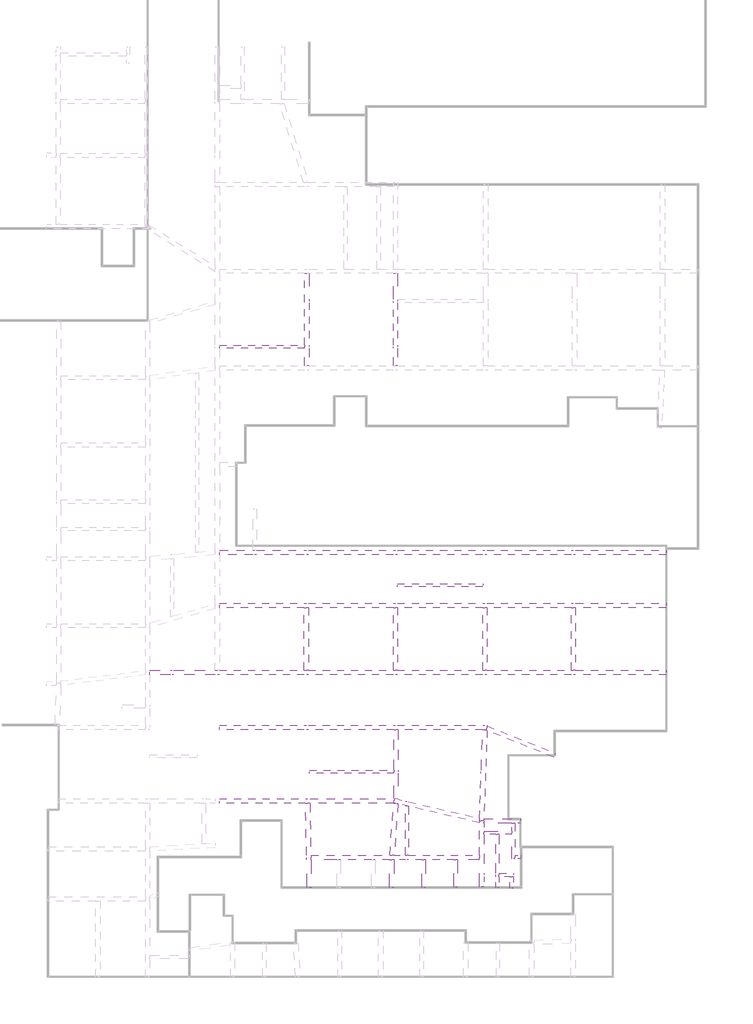
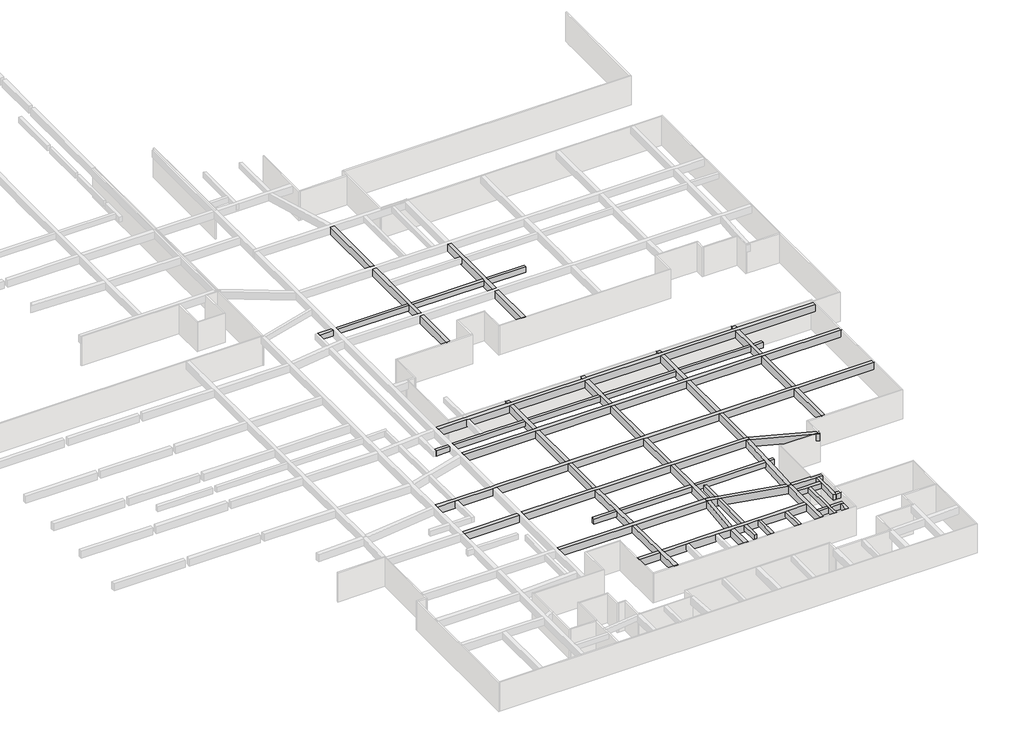
# One storey, part 10 of 16: 33 beams.
"""IFC4 building model written with IfcOpenShell, lengths in millimetres."""

from ifc_helpers import new_model, si_unit, frame, origin, place, context, project, spatial, polyline, outline, extrude, faceted_brep, element, save

model = new_model("IFC4")

# Units and contexts
model_context = context("Model", 3, world=origin())
ifc_project = project(units=[si_unit("LENGTHUNIT", "METRE", prefix="MILLI")], contexts=[model_context])

# Site, building, storey
site = spatial("IfcSite", under=ifc_project)
building = spatial("IfcBuilding", under=site)
storey = spatial("IfcBuildingStorey", under=building, Name="户型图", Elevation=0.0)

# Beams
placement = place(None, origin())
element("IfcBeam", 1, ObjectType="混凝土 - 矩形梁 : KL_beam", at=placement, inside=storey, context=model_context, shape_type="Brep", body=[
    faceted_brep([(196655.472134, 110111.2603451, 3300.0), (196255.472134, 110111.2603451, 3300.0), (196255.472134, 110111.2603451, 2500.0), (196655.472134, 110111.2603451, 2500.0), (196655.472134, 115130.098028, 3300.0), (196255.472134, 115130.098028, 3300.0), (196255.472134, 115130.098028, 2500.0), (196655.472134, 115130.098028, 2500.0)], [[[0, 1, 2, 3]], [[1, 0, 4, 5]], [[2, 1, 5, 6]], [[3, 2, 6, 7]], [[0, 3, 7, 4]], [[5, 4, 7, 6]]]),
    faceted_brep([(196255.472134, 123932.2101355, 3300.0), (196655.472134, 123932.2101355, 3300.0), (196655.472134, 123932.2101355, 2500.0), (196255.472134, 123932.2101355, 2500.0), (196655.472134, 115530.098028, 3300.0), (196255.472134, 115530.098028, 3300.0), (196255.472134, 115530.098028, 2500.0), (196655.472134, 115530.098028, 2500.0), (196255.472134, 117415.9096032, 3300.0), (196255.472134, 117115.9096032, 3300.0), (196655.472134, 117115.9096032, 3300.0), (196655.472134, 117415.9096032, 3300.0), (196655.472134, 121262.5884701, 3300.0), (196655.472134, 121562.5884701, 3300.0)], [[[0, 1, 2, 3]], [[4, 5, 6, 7]], [[1, 0, 8, 9, 5, 4, 10, 11, 12, 13]], [[0, 3, 6, 5, 9, 8]], [[3, 2, 7, 6]], [[2, 1, 13, 12, 11, 10, 4, 7]]]),
    faceted_brep([(196655.472134, 124332.2101355, 3300.0), (196255.472134, 124332.2101355, 3300.0), (196255.472134, 124332.2101355, 2500.0), (196655.472134, 124332.2101355, 2500.0), (196655.472134, 131811.3072201, 3300.0), (196255.472134, 131811.3072201, 3300.0), (196255.472134, 131811.3072201, 2500.0), (196655.472134, 131811.3072201, 2500.0)], [[[0, 1, 2, 3]], [[1, 0, 4, 5]], [[2, 1, 5, 6]], [[3, 2, 6, 7]], [[0, 3, 7, 4]], [[5, 4, 7, 6]]]),
])
element("IfcBeam", 2, ObjectType="混凝土 - 矩形梁 : KL_beam", at=placement, inside=storey, context=model_context, shape_type="Brep", body=[
    faceted_brep([(204716.2109037, 110061.7113145, 3300.0), (204316.2109037, 110061.7113145, 3300.0), (204316.2109037, 110061.7113145, 2500.0), (204716.2109037, 110061.7113145, 2500.0), (204716.2109037, 115130.098028, 3300.0), (204316.2109037, 115130.098028, 3300.0), (204316.2109037, 115130.098028, 2500.0), (204716.2109037, 115130.098028, 2500.0)], [[[0, 1, 2, 3]], [[1, 0, 4, 5]], [[2, 1, 5, 6]], [[3, 2, 6, 7]], [[0, 3, 7, 4]], [[5, 4, 7, 6]]]),
    faceted_brep([(204316.2109037, 123932.2101355, 3300.0), (204716.2109037, 123932.2101355, 3300.0), (204716.2109037, 123932.2101355, 2500.0), (204316.2109037, 123932.2101355, 2500.0), (204716.2109037, 115530.098028, 3300.0), (204316.2109037, 115530.098028, 3300.0), (204316.2109037, 115530.098028, 2500.0), (204716.2109037, 115530.098028, 2500.0), (204316.2109037, 121562.5884701, 3300.0), (204316.2109037, 121262.5884701, 3300.0), (204316.2109037, 117415.9096032, 3300.0), (204316.2109037, 117115.9096032, 3300.0), (204716.2109037, 117115.9096032, 3300.0), (204716.2109037, 117415.9096032, 3300.0), (204716.2109037, 121262.5884701, 3300.0), (204716.2109037, 121562.5884701, 3300.0)], [[[0, 1, 2, 3]], [[4, 5, 6, 7]], [[1, 0, 8, 9, 10, 11, 5, 4, 12, 13, 14, 15]], [[0, 3, 6, 5, 11, 10, 9, 8]], [[3, 2, 7, 6]], [[2, 1, 15, 14, 13, 12, 4, 7]]]),
])
element("IfcBeam", 3, ObjectType="混凝土 - 矩形梁 : KL_beam", at=placement, inside=storey, context=model_context, shape_type="Brep", body=[
    faceted_brep([(229165.989453, 87831.9011327, 3300.0), (229165.989453, 87431.9011327, 3300.0), (229165.989453, 87431.9011327, 2500.0), (229165.989453, 87831.9011327, 2500.0), (220916.2109037, 87831.9011327, 3300.0), (220516.2109037, 87831.9011327, 3300.0), (212857.7367524, 87831.9011327, 3300.0), (212457.7367524, 87831.9011327, 3300.0), (204716.2109037, 87831.9011327, 3300.0), (204316.2109037, 87831.9011327, 3300.0), (196616.2109037, 87831.9011327, 3300.0), (196216.2109037, 87831.9011327, 3300.0), (188516.2109037, 87831.9011327, 3300.0), (188116.2109037, 87831.9011327, 3300.0), (184337.9237533, 87831.9011327, 3300.0), (184037.9237533, 87831.9011327, 3300.0), (182157.7367524, 87831.9011327, 3300.0), (182157.7367524, 87431.9011327, 3300.0), (184037.9237533, 87431.9011327, 3300.0), (184337.9237533, 87431.9011327, 3300.0), (188116.2109037, 87431.9011327, 3300.0), (188516.2109037, 87431.9011327, 3300.0), (196216.2109037, 87431.9011327, 3300.0), (196616.2109037, 87431.9011327, 3300.0), (204316.2109037, 87431.9011327, 3300.0), (204716.2109037, 87431.9011327, 3300.0), (212457.7367524, 87431.9011327, 3300.0), (212857.7367524, 87431.9011327, 3300.0), (220516.2109037, 87431.9011327, 3300.0), (220916.2109037, 87431.9011327, 3300.0), (182157.7367524, 87431.9011327, 2500.0), (188116.2109037, 87431.9011327, 2500.0), (188516.2109037, 87431.9011327, 2500.0), (196216.2109037, 87431.9011327, 2500.0), (196616.2109037, 87431.9011327, 2500.0), (204316.2109037, 87431.9011327, 2500.0), (204716.2109037, 87431.9011327, 2500.0), (212457.7367524, 87431.9011327, 2500.0), (212857.7367524, 87431.9011327, 2500.0), (220516.2109037, 87431.9011327, 2500.0), (220916.2109037, 87431.9011327, 2500.0), (182157.7367524, 87831.9011327, 2500.0), (188116.2109037, 87831.9011327, 2500.0), (188516.2109037, 87831.9011327, 2500.0), (196216.2109037, 87831.9011327, 2500.0), (196616.2109037, 87831.9011327, 2500.0), (204316.2109037, 87831.9011327, 2500.0), (204716.2109037, 87831.9011327, 2500.0), (212457.7367524, 87831.9011327, 2500.0), (212857.7367524, 87831.9011327, 2500.0), (220516.2109037, 87831.9011327, 2500.0), (220916.2109037, 87831.9011327, 2500.0)], [[[0, 1, 2, 3]], [[1, 0, 4, 5, 6, 7, 8, 9, 10, 11, 12, 13, 14, 15, 16, 17, 18, 19, 20, 21, 22, 23, 24, 25, 26, 27, 28, 29]], [[2, 1, 29, 28, 27, 26, 25, 24, 23, 22, 21, 20, 19, 18, 17, 30, 31, 32, 33, 34, 35, 36, 37, 38, 39, 40]], [[3, 2, 40, 39, 38, 37, 36, 35, 34, 33, 32, 31, 30, 41, 42, 43, 44, 45, 46, 47, 48, 49, 50, 51]], [[0, 3, 51, 50, 49, 48, 47, 46, 45, 44, 43, 42, 41, 16, 15, 14, 13, 12, 11, 10, 9, 8, 7, 6, 5, 4]], [[17, 16, 41, 30]]]),
])
element("IfcBeam", 4, ObjectType="混凝土 - 矩形梁 : KL_beam", at=placement, inside=storey, context=model_context, shape_type="Brep", body=[
    faceted_brep([(229166.3202787, 93928.4104182, 3300.0), (229166.3202787, 93528.4104182, 3300.0), (229166.3202787, 93528.4104182, 2500.0), (229166.3202787, 93928.4104182, 2500.0), (220916.2109037, 93928.4104182, 3300.0), (220516.2109037, 93928.4104182, 3300.0), (212857.7367524, 93928.4104182, 3300.0), (212457.7367524, 93928.4104182, 3300.0), (204716.2109037, 93928.4104182, 3300.0), (204316.2109037, 93928.4104182, 3300.0), (196616.2109037, 93928.4104182, 3300.0), (196216.2109037, 93928.4104182, 3300.0), (188516.2109037, 93928.4104182, 3300.0), (188516.2109037, 93528.4104182, 3300.0), (196216.2109037, 93528.4104182, 3300.0), (196616.2109037, 93528.4104182, 3300.0), (204316.2109037, 93528.4104182, 3300.0), (204716.2109037, 93528.4104182, 3300.0), (212457.7367524, 93528.4104182, 3300.0), (212857.7367524, 93528.4104182, 3300.0), (220516.2109037, 93528.4104182, 3300.0), (220916.2109037, 93528.4104182, 3300.0), (188516.2109037, 93528.4104182, 2500.0), (196216.2109037, 93528.4104182, 2500.0), (196616.2109037, 93528.4104182, 2500.0), (204316.2109037, 93528.4104182, 2500.0), (204716.2109037, 93528.4104182, 2500.0), (212457.7367524, 93528.4104182, 2500.0), (212857.7367524, 93528.4104182, 2500.0), (220516.2109037, 93528.4104182, 2500.0), (220916.2109037, 93528.4104182, 2500.0), (188516.2109037, 93928.4104182, 2500.0), (196216.2109037, 93928.4104182, 2500.0), (196616.2109037, 93928.4104182, 2500.0), (204316.2109037, 93928.4104182, 2500.0), (204716.2109037, 93928.4104182, 2500.0), (212457.7367524, 93928.4104182, 2500.0), (212857.7367524, 93928.4104182, 2500.0), (220516.2109037, 93928.4104182, 2500.0), (220916.2109037, 93928.4104182, 2500.0)], [[[0, 1, 2, 3]], [[1, 0, 4, 5, 6, 7, 8, 9, 10, 11, 12, 13, 14, 15, 16, 17, 18, 19, 20, 21]], [[2, 1, 21, 20, 19, 18, 17, 16, 15, 14, 13, 22, 23, 24, 25, 26, 27, 28, 29, 30]], [[3, 2, 30, 29, 28, 27, 26, 25, 24, 23, 22, 31, 32, 33, 34, 35, 36, 37, 38, 39]], [[0, 3, 39, 38, 37, 36, 35, 34, 33, 32, 31, 12, 11, 10, 9, 8, 7, 6, 5, 4]], [[12, 31, 22, 13]]]),
])
element("IfcBeam", 5, ObjectType="混凝土 - 矩形梁 : KL_beam", at=placement, inside=storey, context=model_context, shape_type="Brep", body=[
    faceted_brep([(229166.2265287, 98740.0727237, 3300.0), (229166.2265287, 98340.0727237, 3300.0), (229166.2265287, 98340.0727237, 2500.0), (229166.2265287, 98740.0727237, 2500.0), (220916.2109037, 98740.0727237, 3300.0), (220516.2109037, 98740.0727237, 3300.0), (212857.7367524, 98740.0727237, 3300.0), (212457.7367524, 98740.0727237, 3300.0), (204716.2109037, 98740.0727237, 3300.0), (204316.2109037, 98740.0727237, 3300.0), (196616.2109037, 98740.0727237, 3300.0), (196216.2109037, 98740.0727237, 3300.0), (191866.2868684, 98740.0727237, 3300.0), (191566.2868684, 98740.0727237, 3300.0), (188516.2109037, 98740.0727237, 3300.0), (188516.2109037, 98340.0727237, 3300.0), (191566.2868684, 98340.0727237, 3300.0), (191866.2868684, 98340.0727237, 3300.0), (196216.2109037, 98340.0727237, 3300.0), (196616.2109037, 98340.0727237, 3300.0), (204316.2109037, 98340.0727237, 3300.0), (204716.2109037, 98340.0727237, 3300.0), (212457.7367524, 98340.0727237, 3300.0), (212857.7367524, 98340.0727237, 3300.0), (220516.2109037, 98340.0727237, 3300.0), (220916.2109037, 98340.0727237, 3300.0), (188516.2109037, 98340.0727237, 2500.0), (196216.2109037, 98340.0727237, 2500.0), (196616.2109037, 98340.0727237, 2500.0), (204316.2109037, 98340.0727237, 2500.0), (204716.2109037, 98340.0727237, 2500.0), (212457.7367524, 98340.0727237, 2500.0), (212857.7367524, 98340.0727237, 2500.0), (220516.2109037, 98340.0727237, 2500.0), (220916.2109037, 98340.0727237, 2500.0), (188516.2109037, 98740.0727237, 2500.0), (196216.2109037, 98740.0727237, 2500.0), (196616.2109037, 98740.0727237, 2500.0), (204316.2109037, 98740.0727237, 2500.0), (204716.2109037, 98740.0727237, 2500.0), (212457.7367524, 98740.0727237, 2500.0), (212857.7367524, 98740.0727237, 2500.0), (220516.2109037, 98740.0727237, 2500.0), (220916.2109037, 98740.0727237, 2500.0)], [[[0, 1, 2, 3]], [[1, 0, 4, 5, 6, 7, 8, 9, 10, 11, 12, 13, 14, 15, 16, 17, 18, 19, 20, 21, 22, 23, 24, 25]], [[2, 1, 25, 24, 23, 22, 21, 20, 19, 18, 17, 16, 15, 26, 27, 28, 29, 30, 31, 32, 33, 34]], [[3, 2, 34, 33, 32, 31, 30, 29, 28, 27, 26, 35, 36, 37, 38, 39, 40, 41, 42, 43]], [[0, 3, 43, 42, 41, 40, 39, 38, 37, 36, 35, 14, 13, 12, 11, 10, 9, 8, 7, 6, 5, 4]], [[14, 35, 26, 15]]]),
])
element("IfcBeam", 6, ObjectType="混凝土 - 矩形梁 : KL_beam", at=placement, inside=storey, context=model_context, shape_type="Brep", body=[
    faceted_brep([(212857.7367524, 82438.0259701, 3300.0), (212857.7367524, 82773.7000033, 3300.0), (212857.7367524, 82838.0259701, 3300.0), (212457.7367524, 82838.0259701, 3300.0), (204716.2109037, 82838.0259701, 3300.0), (204316.2109037, 82838.0259701, 3300.0), (196616.2109037, 82838.0259701, 3300.0), (196216.2109037, 82838.0259701, 3300.0), (188516.2109037, 82838.0259701, 3300.0), (188516.2109037, 82438.0259701, 3300.0), (196219.671451, 82438.0259701, 3300.0), (196619.7323823, 82438.0259701, 3300.0), (204365.5652507, 82438.0259701, 3300.0), (204765.5652507, 82438.0259701, 3300.0), (212450.6306897, 82438.0259701, 3300.0), (212619.4103045, 82438.0259701, 3300.0), (212857.7367524, 82438.0259701, 2500.0), (188516.2109037, 82438.0259701, 2500.0), (196219.671451, 82438.0259701, 2500.0), (196619.7323823, 82438.0259701, 2500.0), (204365.5652507, 82438.0259701, 2500.0), (204765.5652507, 82438.0259701, 2500.0), (212450.6306897, 82438.0259701, 2500.0), (212619.4103045, 82438.0259701, 2500.0), (212857.7367524, 82838.0259701, 2500.0), (212857.7367524, 82773.7000033, 2500.0), (188516.2109037, 82838.0259701, 2500.0), (196216.2109037, 82838.0259701, 2500.0), (196616.2109037, 82838.0259701, 2500.0), (204316.2109037, 82838.0259701, 2500.0), (204716.2109037, 82838.0259701, 2500.0), (212457.7367524, 82838.0259701, 2500.0)], [[[0, 1, 2, 3, 4, 5, 6, 7, 8, 9, 10, 11, 12, 13, 14, 15]], [[16, 0, 15, 14, 13, 12, 11, 10, 9, 17, 18, 19, 20, 21, 22, 23]], [[24, 25, 16, 23, 22, 21, 20, 19, 18, 17, 26, 27, 28, 29, 30, 31]], [[2, 24, 31, 30, 29, 28, 27, 26, 8, 7, 6, 5, 4, 3]], [[9, 8, 26, 17]], [[2, 1, 0, 16, 25, 24]]]),
    faceted_brep([(182157.7367524, 82438.0259701, 3300.0), (182157.7367524, 82838.0259701, 3300.0), (182157.7367524, 82838.0259701, 2500.0), (182157.7367524, 82438.0259701, 2500.0), (188116.2109037, 82838.0259701, 3300.0), (188116.2109037, 82438.0259701, 3300.0), (188116.2109037, 82438.0259701, 2500.0), (188116.2109037, 82838.0259701, 2500.0)], [[[0, 1, 2, 3]], [[4, 5, 6, 7]], [[1, 0, 5, 4]], [[0, 3, 6, 5]], [[3, 2, 7, 6]], [[2, 1, 4, 7]]]),
])
element("IfcBeam", 7, ObjectType="混凝土 - 矩形梁 : KL_beam", at=placement, inside=storey, context=model_context, shape_type="Brep", body=[
    faceted_brep([(196216.2109037, 99161.1613461, 3300.0), (196616.2109037, 99161.1613461, 3300.0), (196616.2109037, 99161.1613461, 2500.0), (196216.2109037, 99161.1613461, 2500.0), (196216.2109037, 98740.0727237, 3300.0), (196616.2109037, 98740.0727237, 3300.0), (196616.2109037, 98740.0727237, 2500.0), (196216.2109037, 98740.0727237, 2500.0)], [[[0, 1, 2, 3]], [[1, 0, 4, 5]], [[2, 1, 5, 6]], [[3, 2, 6, 7]], [[0, 3, 7, 4]], [[5, 4, 7, 6]]]),
    faceted_brep([(196616.2109037, 82838.0259701, 3300.0), (196216.2109037, 82838.0259701, 3300.0), (196216.2109037, 82838.0259701, 2500.0), (196616.2109037, 82838.0259701, 2500.0), (196216.2109037, 87431.9011327, 3300.0), (196616.2109037, 87431.9011327, 3300.0), (196616.2109037, 87431.9011327, 2500.0), (196216.2109037, 87431.9011327, 2500.0)], [[[0, 1, 2, 3]], [[4, 5, 6, 7]], [[1, 0, 5, 4]], [[0, 3, 6, 5]], [[3, 2, 7, 6]], [[2, 1, 4, 7]]]),
    faceted_brep([(196616.2109037, 87831.9011327, 3300.0), (196216.2109037, 87831.9011327, 3300.0), (196216.2109037, 87831.9011327, 2500.0), (196616.2109037, 87831.9011327, 2500.0), (196216.2109037, 93528.4104182, 3300.0), (196616.2109037, 93528.4104182, 3300.0), (196616.2109037, 93528.4104182, 2500.0), (196216.2109037, 93528.4104182, 2500.0)], [[[0, 1, 2, 3]], [[4, 5, 6, 7]], [[1, 0, 5, 4]], [[0, 3, 6, 5]], [[3, 2, 7, 6]], [[2, 1, 4, 7]]]),
    faceted_brep([(196616.2109037, 93928.4104182, 3300.0), (196216.2109037, 93928.4104182, 3300.0), (196216.2109037, 93928.4104182, 2500.0), (196616.2109037, 93928.4104182, 2500.0), (196216.2109037, 98340.0727237, 3300.0), (196616.2109037, 98340.0727237, 3300.0), (196616.2109037, 98340.0727237, 2500.0), (196216.2109037, 98340.0727237, 2500.0), (196616.2109037, 95415.9096032, 3300.0), (196616.2109037, 95715.9096032, 3300.0), (196216.2109037, 95715.9096032, 3300.0), (196216.2109037, 95415.9096032, 3300.0)], [[[0, 1, 2, 3]], [[4, 5, 6, 7]], [[1, 0, 8, 9, 5, 4, 10, 11]], [[0, 3, 6, 5, 9, 8]], [[3, 2, 7, 6]], [[2, 1, 11, 10, 4, 7]]]),
])
element("IfcBeam", 8, ObjectType="混凝土 - 矩形梁 : KL_beam", at=placement, inside=storey, context=model_context, shape_type="Brep", body=[
    faceted_brep([(204316.2109037, 99161.1613461, 3300.0), (204716.2109037, 99161.1613461, 3300.0), (204716.2109037, 99161.1613461, 2500.0), (204316.2109037, 99161.1613461, 2500.0), (204316.2109037, 98740.0727237, 3300.0), (204716.2109037, 98740.0727237, 3300.0), (204716.2109037, 98740.0727237, 2500.0), (204316.2109037, 98740.0727237, 2500.0)], [[[0, 1, 2, 3]], [[1, 0, 4, 5]], [[2, 1, 5, 6]], [[3, 2, 6, 7]], [[0, 3, 7, 4]], [[5, 4, 7, 6]]]),
    faceted_brep([(204716.2109037, 82838.0259701, 3300.0), (204316.2109037, 82838.0259701, 3300.0), (204316.2109037, 82838.0259701, 2500.0), (204716.2109037, 82838.0259701, 2500.0), (204316.2109037, 87431.9011327, 3300.0), (204716.2109037, 87431.9011327, 3300.0), (204716.2109037, 87431.9011327, 2500.0), (204316.2109037, 87431.9011327, 2500.0)], [[[0, 1, 2, 3]], [[4, 5, 6, 7]], [[1, 0, 5, 4]], [[0, 3, 6, 5]], [[3, 2, 7, 6]], [[2, 1, 4, 7]]]),
    faceted_brep([(204716.2109037, 87831.9011327, 3300.0), (204316.2109037, 87831.9011327, 3300.0), (204316.2109037, 87831.9011327, 2500.0), (204716.2109037, 87831.9011327, 2500.0), (204316.2109037, 93528.4104182, 3300.0), (204716.2109037, 93528.4104182, 3300.0), (204716.2109037, 93528.4104182, 2500.0), (204316.2109037, 93528.4104182, 2500.0)], [[[0, 1, 2, 3]], [[4, 5, 6, 7]], [[1, 0, 5, 4]], [[0, 3, 6, 5]], [[3, 2, 7, 6]], [[2, 1, 4, 7]]]),
    faceted_brep([(204716.2109037, 93928.4104182, 3300.0), (204316.2109037, 93928.4104182, 3300.0), (204316.2109037, 93928.4104182, 2500.0), (204716.2109037, 93928.4104182, 2500.0), (204316.2109037, 98340.0727237, 3300.0), (204716.2109037, 98340.0727237, 3300.0), (204716.2109037, 98340.0727237, 2500.0), (204316.2109037, 98340.0727237, 2500.0), (204716.2109037, 95415.9096032, 3300.0), (204716.2109037, 95715.9096032, 3300.0), (204316.2109037, 95715.9096032, 3300.0), (204316.2109037, 95415.9096032, 3300.0)], [[[0, 1, 2, 3]], [[4, 5, 6, 7]], [[1, 0, 8, 9, 5, 4, 10, 11]], [[0, 3, 6, 5, 9, 8]], [[3, 2, 7, 6]], [[2, 1, 11, 10, 4, 7]]]),
])
element("IfcBeam", 9, ObjectType="混凝土 - 矩形梁 : KL_beam", at=placement, inside=storey, context=model_context, shape_type="Brep", body=[
    faceted_brep([(212457.7367524, 99161.1665951, 3300.0), (212857.7367524, 99161.1665951, 3300.0), (212857.7367524, 99161.1665951, 2500.0), (212457.7367524, 99161.1665951, 2500.0), (212457.7367524, 98740.0727237, 3300.0), (212857.7367524, 98740.0727237, 3300.0), (212857.7367524, 98740.0727237, 2500.0), (212457.7367524, 98740.0727237, 2500.0)], [[[0, 1, 2, 3]], [[1, 0, 4, 5]], [[2, 1, 5, 6]], [[3, 2, 6, 7]], [[0, 3, 7, 4]], [[5, 4, 7, 6]]]),
    faceted_brep([(212857.7367524, 82838.0259701, 3300.0), (212457.7367524, 82838.0259701, 3300.0), (212457.7367524, 82838.0259701, 2500.0), (212857.7367524, 82838.0259701, 2500.0), (212457.7367524, 87431.9011327, 3300.0), (212857.7367524, 87431.9011327, 3300.0), (212857.7367524, 87431.9011327, 2500.0), (212457.7367524, 87431.9011327, 2500.0)], [[[0, 1, 2, 3]], [[4, 5, 6, 7]], [[1, 0, 5, 4]], [[0, 3, 6, 5]], [[3, 2, 7, 6]], [[2, 1, 4, 7]]]),
    faceted_brep([(212857.7367524, 87831.9011327, 3300.0), (212457.7367524, 87831.9011327, 3300.0), (212457.7367524, 87831.9011327, 2500.0), (212857.7367524, 87831.9011327, 2500.0), (212457.7367524, 93528.4104182, 3300.0), (212857.7367524, 93528.4104182, 3300.0), (212857.7367524, 93528.4104182, 2500.0), (212457.7367524, 93528.4104182, 2500.0)], [[[0, 1, 2, 3]], [[4, 5, 6, 7]], [[1, 0, 5, 4]], [[0, 3, 6, 5]], [[3, 2, 7, 6]], [[2, 1, 4, 7]]]),
    faceted_brep([(212857.7367524, 93928.4104182, 3300.0), (212457.7367524, 93928.4104182, 3300.0), (212457.7367524, 93928.4104182, 2500.0), (212857.7367524, 93928.4104182, 2500.0), (212457.7367524, 98340.0727237, 3300.0), (212857.7367524, 98340.0727237, 3300.0), (212857.7367524, 98340.0727237, 2500.0), (212457.7367524, 98340.0727237, 2500.0), (212857.7367524, 95415.9096032, 3300.0), (212857.7367524, 95715.9096032, 3300.0), (212457.7367524, 95715.9096032, 3300.0), (212457.7367524, 95415.9096032, 3300.0)], [[[0, 1, 2, 3]], [[4, 5, 6, 7]], [[1, 0, 8, 9, 5, 4, 10, 11]], [[0, 3, 6, 5, 9, 8]], [[3, 2, 7, 6]], [[2, 1, 11, 10, 4, 7]]]),
])
element("IfcBeam", 10, ObjectType="混凝土 - 矩形梁 : KL_beam", at=placement, inside=storey, context=model_context, shape_type="Brep", body=[
    faceted_brep([(220516.2109037, 99161.2550961, 3300.0), (220916.2109037, 99161.2550961, 3300.0), (220916.2109037, 99161.2550961, 2500.0), (220516.2109037, 99161.2550961, 2500.0), (220516.2109037, 98740.0727237, 3300.0), (220916.2109037, 98740.0727237, 3300.0), (220916.2109037, 98740.0727237, 2500.0), (220516.2109037, 98740.0727237, 2500.0)], [[[0, 1, 2, 3]], [[1, 0, 4, 5]], [[2, 1, 5, 6]], [[3, 2, 6, 7]], [[0, 3, 7, 4]], [[5, 4, 7, 6]]]),
    faceted_brep([(220516.2109037, 82302.2550961, 3300.0), (220516.2109037, 82302.2550961, 2500.0), (220916.2109037, 82302.2550961, 2500.0), (220916.2109037, 82302.2550961, 3300.0), (220516.2109037, 87431.9011327, 3300.0), (220916.2109037, 87431.9011327, 3300.0), (220916.2109037, 87431.9011327, 2500.0), (220516.2109037, 87431.9011327, 2500.0)], [[[0, 1, 2, 3]], [[4, 5, 6, 7]], [[0, 3, 5, 4]], [[3, 2, 6, 5]], [[2, 1, 7, 6]], [[1, 0, 4, 7]]]),
    faceted_brep([(220916.2109037, 87831.9011327, 3300.0), (220516.2109037, 87831.9011327, 3300.0), (220516.2109037, 87831.9011327, 2500.0), (220916.2109037, 87831.9011327, 2500.0), (220516.2109037, 93528.4104182, 3300.0), (220916.2109037, 93528.4104182, 3300.0), (220916.2109037, 93528.4104182, 2500.0), (220516.2109037, 93528.4104182, 2500.0)], [[[0, 1, 2, 3]], [[4, 5, 6, 7]], [[1, 0, 5, 4]], [[0, 3, 6, 5]], [[3, 2, 7, 6]], [[2, 1, 4, 7]]]),
    faceted_brep([(220916.2109037, 93928.4104182, 3300.0), (220516.2109037, 93928.4104182, 3300.0), (220516.2109037, 93928.4104182, 2500.0), (220916.2109037, 93928.4104182, 2500.0), (220516.2109037, 98340.0727237, 3300.0), (220916.2109037, 98340.0727237, 3300.0), (220916.2109037, 98340.0727237, 2500.0), (220516.2109037, 98340.0727237, 2500.0), (220916.2109037, 95415.9096032, 3300.0), (220916.2109037, 95715.9096032, 3300.0), (220516.2109037, 95715.9096032, 3300.0), (220516.2109037, 95415.9096032, 3300.0)], [[[0, 1, 2, 3]], [[4, 5, 6, 7]], [[1, 0, 8, 9, 5, 4, 10, 11]], [[0, 3, 6, 5, 9, 8]], [[3, 2, 7, 6]], [[2, 1, 11, 10, 4, 7]]]),
])
element("IfcBeam", 11, ObjectType="混凝土 - 矩形梁 : KL_beam", at=placement, inside=storey, context=model_context, shape_type="Brep", body=[
    faceted_brep([(219079.6758919, 80298.142032, 3300.0), (218931.8005151, 79926.4797217, 3300.0), (218931.8005151, 79926.4797217, 2500.0), (219079.6758919, 80298.142032, 2500.0), (212857.7367524, 82773.7000033, 3300.0), (212857.7367524, 82438.0259701, 3300.0), (212619.4103045, 82438.0259701, 3300.0), (212847.7025863, 82347.1940341, 3300.0), (212619.4103045, 82438.0259701, 2500.0), (212847.7025863, 82347.1940341, 2500.0), (212857.7367524, 82438.0259701, 2500.0), (212857.7367524, 82773.7000033, 2500.0)], [[[0, 1, 2, 3]], [[1, 0, 4, 5, 6, 7]], [[2, 1, 7, 6, 8, 9]], [[3, 2, 9, 8, 10, 11]], [[0, 3, 11, 4]], [[5, 10, 8, 6]], [[10, 5, 4, 11]]]),
])
element("IfcBeam", 12, ObjectType="混凝土 - 矩形梁 : KL_beam", at=placement, inside=storey, context=model_context, shape_type="Brep", body=[
    faceted_brep([(212450.6306897, 82438.0259701, 3300.0), (212321.9177065, 78752.1683832, 3300.0), (212311.4414756, 78452.1683832, 3300.0), (212169.1148986, 74376.4684731, 3300.0), (212160.525769, 74130.5079832, 3300.0), (212560.525769, 74123.5259572, 3300.0), (212567.6318318, 74327.0169702, 3300.0), (212711.6852934, 78452.1683832, 3300.0), (212722.1615242, 78752.1683832, 3300.0), (212847.7025863, 82347.1940341, 3300.0), (212619.4103045, 82438.0259701, 3300.0), (212457.7367524, 82438.0259701, 3300.0), (212450.6306897, 82438.0259701, 2500.0), (212169.1148986, 74376.4684731, 2500.0), (212160.525769, 74130.5079832, 2500.0), (212457.7367524, 82438.0259701, 2500.0), (212619.4103045, 82438.0259701, 2500.0), (212847.7025863, 82347.1940341, 2500.0), (212567.6318318, 74327.0169702, 2500.0), (212560.525769, 74123.5259572, 2500.0)], [[[0, 1, 2, 3, 4, 5, 6, 7, 8, 9, 10, 11]], [[4, 3, 2, 1, 0, 12, 13, 14]], [[14, 13, 12, 15, 16, 17, 18, 19]], [[5, 19, 18, 17, 9, 8, 7, 6]], [[12, 0, 11, 10, 16, 15]], [[10, 9, 17, 16]], [[5, 4, 14, 19]]]),
])
element("IfcBeam", 13, ObjectType="混凝土 - 矩形梁 : KL_beam", at=placement, inside=storey, context=model_context, shape_type="Brep", body=[
    faceted_brep([(212560.525769, 68162.6620951, 3300.0), (212160.525769, 68162.6620951, 3300.0), (212160.525769, 68162.6620951, 2500.0), (212560.525769, 68162.6620951, 2500.0), (212560.525769, 69072.3236201, 3300.0), (212560.525769, 69372.3236201, 3300.0), (212560.525769, 72912.3072201, 3300.0), (212560.525769, 73212.3072201, 3300.0), (212560.525769, 73927.0169702, 3300.0), (212560.525769, 74123.5259572, 3300.0), (212160.525769, 74130.5079832, 3300.0), (212160.525769, 73967.9297868, 3300.0), (212160.525769, 71002.3072201, 3300.0), (212160.525769, 70602.3072201, 3300.0), (212160.525769, 74130.5079832, 2500.0), (212160.525769, 73967.9297868, 2500.0), (212160.525769, 71002.3072201, 2500.0), (212160.525769, 70602.3072201, 2500.0), (212560.525769, 74123.5259572, 2500.0), (212560.525769, 73927.0169702, 2500.0)], [[[0, 1, 2, 3]], [[1, 0, 4, 5, 6, 7, 8, 9, 10, 11, 12, 13]], [[2, 1, 13, 12, 11, 10, 14, 15, 16, 17]], [[3, 2, 17, 16, 15, 14, 18, 19]], [[0, 3, 19, 18, 9, 8, 7, 6, 5, 4]], [[9, 18, 14, 10]]]),
])
element("IfcBeam", 14, ObjectType="混凝土 - 矩形梁 : KL_beam", at=placement, inside=storey, context=model_context, shape_type="Brep", body=[
    faceted_brep([(212160.525769, 74130.5079832, 3300.0), (212169.1148986, 74376.4684731, 3300.0), (205715.469601, 75866.4098892, 3300.0), (205415.469601, 75935.6703465, 3300.0), (204765.5652507, 76085.7125882, 3300.0), (204365.5652507, 76178.0598647, 3300.0), (204365.5652507, 76126.6254049, 3300.0), (204365.5652507, 75767.5382216, 3300.0), (204542.7781291, 75726.6254049, 3300.0), (204747.7405268, 75679.3061069, 3300.0), (205415.469601, 75525.1487034, 3300.0), (205715.469601, 75455.888246, 3300.0), (212160.525769, 73967.9297868, 3300.0), (212169.1148986, 74376.4684731, 2500.0), (204765.5652507, 76085.7125882, 2500.0), (204365.5652507, 76178.0598647, 2500.0), (212160.525769, 74130.5079832, 2500.0), (212160.525769, 73967.9297868, 2500.0), (204747.7405268, 75679.3061069, 2500.0), (204542.7781291, 75726.6254049, 2500.0), (204365.5652507, 75767.5382216, 2500.0), (204365.5652507, 76126.6254049, 2500.0)], [[[0, 1, 2, 3, 4, 5, 6, 7, 8, 9, 10, 11, 12]], [[1, 13, 14, 15, 5, 4, 3, 2]], [[13, 16, 17, 18, 19, 20, 21, 15, 14]], [[7, 20, 19, 18, 17, 12, 11, 10, 9, 8]], [[1, 0, 16, 13]], [[0, 12, 17, 16]], [[7, 6, 5, 15, 21, 20]]]),
])
element("IfcBeam", 15, ObjectType="混凝土 - 矩形梁 : KL_beam", at=placement, inside=storey, context=model_context, shape_type="Brep", body=[
    faceted_brep([(204365.5652507, 76178.0598647, 3300.0), (204765.5652507, 76085.7125882, 3300.0), (204765.5652507, 78452.1683832, 3300.0), (204765.5652507, 78752.1683832, 3300.0), (204765.5652507, 82438.0259701, 3300.0), (204365.5652507, 82438.0259701, 3300.0), (204365.5652507, 78752.1683832, 3300.0), (204365.5652507, 78452.1683832, 3300.0), (204765.5652507, 76085.7125882, 2500.0), (204765.5652507, 82438.0259701, 2500.0), (204365.5652507, 76178.0598647, 2500.0), (204365.5652507, 82438.0259701, 2500.0)], [[[0, 1, 2, 3, 4, 5, 6, 7]], [[1, 8, 9, 4, 3, 2]], [[8, 10, 11, 9]], [[10, 0, 7, 6, 5, 11]], [[1, 0, 10, 8]], [[5, 4, 9, 11]]]),
])
element("IfcBeam", 16, ObjectType="混凝土 - 矩形梁 : KL_beam", at=placement, inside=storey, context=model_context, shape_type="Brep", body=[
    faceted_brep([(204542.7781291, 75726.6254049, 3300.0), (204365.5652507, 75767.5382216, 3300.0), (204365.5652507, 76126.6254049, 3300.0), (196729.8982889, 76126.6254049, 3300.0), (196329.8373577, 76126.6254049, 3300.0), (188516.2109037, 76126.6254049, 3300.0), (188516.2109037, 75726.6254049, 3300.0), (196336.8193837, 75726.6254049, 3300.0), (196736.8803149, 75726.6254049, 3300.0), (204350.1537866, 75726.6254049, 3300.0), (204365.5652507, 76126.6254049, 2500.0), (196729.8982889, 76126.6254049, 2500.0), (196329.8373577, 76126.6254049, 2500.0), (188516.2109037, 76126.6254049, 2500.0), (204365.5652507, 75767.5382216, 2500.0), (204542.7781291, 75726.6254049, 2500.0), (204350.1537866, 75726.6254049, 2500.0), (196736.8803149, 75726.6254049, 2500.0), (196336.8193837, 75726.6254049, 2500.0), (188516.2109037, 75726.6254049, 2500.0)], [[[0, 1, 2, 3, 4, 5, 6, 7, 8, 9]], [[2, 10, 11, 12, 13, 5, 4, 3]], [[14, 15, 16, 17, 18, 19, 13, 12, 11, 10]], [[15, 0, 9, 8, 7, 6, 19, 18, 17, 16]], [[14, 1, 0, 15]], [[1, 14, 10, 2]], [[6, 5, 13, 19]]]),
])
element("IfcBeam", 17, ObjectType="混凝土 - 矩形梁 : KL_beam", at=placement, inside=storey, context=model_context, shape_type="Brep", body=[
    faceted_brep([(196870.5923656, 68066.2671502, 3300.0), (196470.6532875, 68059.2861877, 3300.0), (196470.6532875, 68059.2861877, 2500.0), (196870.5923656, 68066.2671502, 2500.0), (196826.3256215, 70602.3072201, 3300.0), (196819.3435955, 71002.3072201, 3300.0), (196736.8803149, 75726.6254049, 3300.0), (196336.8193837, 75726.6254049, 3300.0), (196419.2826643, 71002.3072201, 3300.0), (196426.2646903, 70602.3072201, 3300.0), (196336.8193837, 75726.6254049, 2500.0), (196419.2826643, 71002.3072201, 2500.0), (196426.2646903, 70602.3072201, 2500.0), (196736.8803149, 75726.6254049, 2500.0), (196819.3435955, 71002.3072201, 2500.0), (196826.3256215, 70602.3072201, 2500.0)], [[[0, 1, 2, 3]], [[1, 0, 4, 5, 6, 7, 8, 9]], [[2, 1, 9, 8, 7, 10, 11, 12]], [[3, 2, 12, 11, 10, 13, 14, 15]], [[0, 3, 15, 14, 13, 6, 5, 4]], [[7, 6, 13, 10]]]),
    faceted_brep([(196219.671451, 82438.0259701, 3300.0), (196619.7323823, 82438.0259701, 3300.0), (196619.7323823, 82438.0259701, 2500.0), (196219.671451, 82438.0259701, 2500.0), (196729.8982889, 76126.6254049, 3300.0), (196329.8373577, 76126.6254049, 3300.0), (196329.8373577, 76126.6254049, 2500.0), (196729.8982889, 76126.6254049, 2500.0), (196284.0083345, 78752.1683832, 3300.0), (196289.244854, 78452.1683832, 3300.0), (196689.3057852, 78452.1683832, 3300.0), (196684.0692657, 78752.1683832, 3300.0)], [[[0, 1, 2, 3]], [[4, 5, 6, 7]], [[1, 0, 8, 9, 5, 4, 10, 11]], [[0, 3, 6, 5, 9, 8]], [[3, 2, 7, 6]], [[2, 1, 11, 10, 4, 7]]]),
])
element("IfcBeam", 18, ObjectType="混凝土 - 矩形梁 : KL_beam", at=placement, inside=storey, context=model_context, shape_type="SweptSolid", body=[
    extrude(outline(polyline([(204542.7781291, 75726.6254049), (204747.7405268, 75679.3061069), (204400.2357023, 71002.3072201), (203999.1330998, 71002.3072201), (204350.1537866, 75726.6254049), (204542.7781291, 75726.6254049)])), frame((0.0, 0.0, 2500.0), z_axis=(0.0, 0.0, 1.0), x_axis=(1.0, 0.0, 0.0)), (0.0, 0.0, 1.0), 800.0),
])
element("IfcBeam", 19, ObjectType="混凝土 - 矩形梁 : KL_beam", at=placement, inside=storey, context=model_context, shape_type="SweptSolid", body=[
    extrude(outline(polyline([(204396.7123685, 68062.3072201), (203996.7123685, 68062.3072201), (203996.7123685, 70602.3072201), (204396.7123685, 70602.3072201), (204396.7123685, 68062.3072201)])), frame((0.0, 0.0, 2500.0), z_axis=(0.0, 0.0, 1.0), x_axis=(1.0, 0.0, 0.0)), (0.0, 0.0, 1.0), 800.0),
])
element("IfcBeam", 20, ObjectType="混凝土 - 矩形梁 : KL_beam", at=placement, inside=storey, context=model_context, shape_type="Brep", body=[
    faceted_brep([(194147.1180922, 71002.3072201, 3300.0), (194147.1180922, 71002.3072201, 2500.0), (194147.1180922, 70602.3072201, 2500.0), (194147.1180922, 70602.3072201, 3300.0), (196419.2826643, 71002.3072201, 3300.0), (196426.2646903, 70602.3072201, 3300.0), (196426.2646903, 70602.3072201, 2500.0), (196419.2826643, 71002.3072201, 2500.0)], [[[0, 1, 2, 3]], [[4, 5, 6, 7]], [[0, 3, 5, 4]], [[3, 2, 6, 5]], [[2, 1, 7, 6]], [[1, 0, 4, 7]]]),
    faceted_brep([(212160.525769, 70602.3072201, 3300.0), (212160.525769, 71002.3072201, 3300.0), (205715.469601, 71002.3072201, 3300.0), (205415.469601, 71002.3072201, 3300.0), (204400.2357023, 71002.3072201, 3300.0), (203999.1330998, 71002.3072201, 3300.0), (196819.3435955, 71002.3072201, 3300.0), (196826.3256215, 70602.3072201, 3300.0), (199196.7123685, 70602.3072201, 3300.0), (199496.7123685, 70602.3072201, 3300.0), (202346.7123685, 70602.3072201, 3300.0), (202646.7123685, 70602.3072201, 3300.0), (203996.7123685, 70602.3072201, 3300.0), (204396.7123685, 70602.3072201, 3300.0), (205415.469601, 70602.3072201, 3300.0), (205715.469601, 70602.3072201, 3300.0), (206946.7123685, 70602.3072201, 3300.0), (207246.7123685, 70602.3072201, 3300.0), (209846.7143216, 70602.3072201, 3300.0), (210146.7143216, 70602.3072201, 3300.0), (212160.525769, 70602.3072201, 2500.0), (196826.3256215, 70602.3072201, 2500.0), (203996.7123685, 70602.3072201, 2500.0), (204396.7123685, 70602.3072201, 2500.0), (212160.525769, 71002.3072201, 2500.0), (196819.3435955, 71002.3072201, 2500.0), (203999.1330998, 71002.3072201, 2500.0), (204400.2357023, 71002.3072201, 2500.0)], [[[0, 1, 2, 3, 4, 5, 6, 7, 8, 9, 10, 11, 12, 13, 14, 15, 16, 17, 18, 19]], [[20, 0, 19, 18, 17, 16, 15, 14, 13, 12, 11, 10, 9, 8, 7, 21, 22, 23]], [[24, 20, 23, 22, 21, 25, 26, 27]], [[1, 24, 27, 26, 25, 6, 5, 4, 3, 2]], [[1, 0, 20, 24]], [[7, 6, 25, 21]]]),
])
element("IfcBeam", 21, ObjectType="混凝土 - 矩形梁 : KL_beam", at=placement, inside=storey, context=model_context, shape_type="Brep", body=[
    faceted_brep([(215896.8214613, 74327.0169702, 3300.0), (215896.8214613, 73927.0169702, 3300.0), (215896.8214613, 73927.0169702, 2500.0), (215896.8214613, 74327.0169702, 2500.0), (212567.6318318, 74327.0169702, 3300.0), (212566.1577194, 74284.8039153, 3300.0), (212560.525769, 74123.5259572, 3300.0), (212560.525769, 73927.0169702, 3300.0), (215096.7143216, 73927.0169702, 3300.0), (215396.7143216, 73927.0169702, 3300.0), (212560.525769, 73927.0169702, 2500.0), (212560.525769, 74123.5259572, 2500.0), (212566.1577194, 74284.8039153, 2500.0), (212567.6318318, 74327.0169702, 2500.0)], [[[0, 1, 2, 3]], [[1, 0, 4, 5, 6, 7, 8, 9]], [[2, 1, 9, 8, 7, 10]], [[3, 2, 10, 11, 12, 13]], [[0, 3, 13, 4]], [[4, 13, 12, 11, 6, 5]], [[7, 6, 11, 10]]]),
])
element("IfcBeam", 22, ObjectType="混凝土 - 矩形梁 : L_beam", at=placement, inside=storey, context=model_context, shape_type="Brep", body=[
    faceted_brep([(221797.6194037, 95715.9096032, 3300.0), (221797.6194037, 95415.9096032, 3300.0), (221797.6194037, 95415.9096032, 2700.0), (221797.6194037, 95715.9096032, 2700.0), (220916.2109037, 95715.9096032, 3300.0), (220916.2109037, 95415.9096032, 3300.0), (220916.2109037, 95415.9096032, 2700.0), (220916.2109037, 95715.9096032, 2700.0)], [[[0, 1, 2, 3]], [[1, 0, 4, 5]], [[2, 1, 5, 6]], [[3, 2, 6, 7]], [[0, 3, 7, 4]], [[5, 4, 7, 6]]]),
    faceted_brep([(186611.3422117, 95415.9096032, 3300.0), (186611.3422117, 95715.9096032, 3300.0), (186611.3422117, 95715.9096032, 2700.0), (186611.3422117, 95415.9096032, 2700.0), (188116.2109037, 95715.9096032, 3300.0), (188116.2109037, 95415.9096032, 3300.0), (188116.2109037, 95415.9096032, 2700.0), (188116.2109037, 95715.9096032, 2700.0)], [[[0, 1, 2, 3]], [[4, 5, 6, 7]], [[1, 0, 5, 4]], [[0, 3, 6, 5]], [[3, 2, 7, 6]], [[2, 1, 4, 7]]]),
    faceted_brep([(188516.2109037, 95415.9096032, 3300.0), (188516.2109037, 95715.9096032, 3300.0), (188516.2109037, 95715.9096032, 2700.0), (188516.2109037, 95415.9096032, 2700.0), (196216.2109037, 95715.9096032, 3300.0), (196216.2109037, 95415.9096032, 3300.0), (196216.2109037, 95415.9096032, 2700.0), (196216.2109037, 95715.9096032, 2700.0), (191866.2868684, 95715.9096032, 3300.0), (191566.2868684, 95715.9096032, 3300.0), (191566.2868684, 95715.9096032, 2700.0), (191866.2868684, 95715.9096032, 2700.0)], [[[0, 1, 2, 3]], [[4, 5, 6, 7]], [[1, 0, 5, 4, 8, 9]], [[0, 3, 6, 5]], [[3, 2, 10, 11, 7, 6]], [[2, 1, 9, 8, 4, 7, 11, 10]]]),
    faceted_brep([(196616.2109037, 95415.9096032, 3300.0), (196616.2109037, 95715.9096032, 3300.0), (196616.2109037, 95715.9096032, 2700.0), (196616.2109037, 95415.9096032, 2700.0), (204316.2109037, 95715.9096032, 3300.0), (204316.2109037, 95415.9096032, 3300.0), (204316.2109037, 95415.9096032, 2700.0), (204316.2109037, 95715.9096032, 2700.0)], [[[0, 1, 2, 3]], [[4, 5, 6, 7]], [[1, 0, 5, 4]], [[0, 3, 6, 5]], [[3, 2, 7, 6]], [[2, 1, 4, 7]]]),
    faceted_brep([(204716.2109037, 95415.9096032, 3300.0), (204716.2109037, 95715.9096032, 3300.0), (204716.2109037, 95715.9096032, 2700.0), (204716.2109037, 95415.9096032, 2700.0), (212457.7367524, 95715.9096032, 3300.0), (212457.7367524, 95415.9096032, 3300.0), (212457.7367524, 95415.9096032, 2700.0), (212457.7367524, 95715.9096032, 2700.0)], [[[0, 1, 2, 3]], [[4, 5, 6, 7]], [[1, 0, 5, 4]], [[0, 3, 6, 5]], [[3, 2, 7, 6]], [[2, 1, 4, 7]]]),
    faceted_brep([(212857.7367524, 95415.9096032, 3300.0), (212857.7367524, 95715.9096032, 3300.0), (212857.7367524, 95715.9096032, 2700.0), (212857.7367524, 95415.9096032, 2700.0), (220516.2109037, 95715.9096032, 3300.0), (220516.2109037, 95415.9096032, 3300.0), (220516.2109037, 95415.9096032, 2700.0), (220516.2109037, 95715.9096032, 2700.0)], [[[0, 1, 2, 3]], [[4, 5, 6, 7]], [[1, 0, 5, 4]], [[0, 3, 6, 5]], [[3, 2, 7, 6]], [[2, 1, 4, 7]]]),
])
element("IfcBeam", 23, ObjectType="混凝土 - 矩形梁 : L_beam", at=placement, inside=storey, context=model_context, shape_type="SweptSolid", body=[
    extrude(outline(polyline([(208785.8300636, 117415.9096032), (208785.8300636, 117115.9096032), (204716.2109037, 117115.9096032), (204716.2109037, 117415.9096032), (208785.8300636, 117415.9096032)])), frame((0.0, 0.0, 2700.0), z_axis=(0.0, 0.0, 1.0), x_axis=(1.0, 0.0, 0.0)), (0.0, 0.0, 1.0), 600.0),
    extrude(outline(polyline([(186611.3422117, 117115.9096032), (186611.3422117, 117415.9096032), (188116.2109037, 117415.9096032), (188116.2109037, 117115.9096032), (186611.3422117, 117115.9096032)])), frame((0.0, 0.0, 2700.0), z_axis=(0.0, 0.0, 1.0), x_axis=(1.0, 0.0, 0.0)), (0.0, 0.0, 1.0), 600.0),
    extrude(outline(polyline([(196255.472134, 117415.9096032), (196255.472134, 117115.9096032), (188516.2109037, 117115.9096032), (188516.2109037, 117415.9096032), (196255.472134, 117415.9096032)])), frame((0.0, 0.0, 2700.0), z_axis=(0.0, 0.0, 1.0), x_axis=(1.0, 0.0, 0.0)), (0.0, 0.0, 1.0), 600.0),
    extrude(outline(polyline([(196655.472134, 117115.9096032), (196655.472134, 117415.9096032), (204316.2109037, 117415.9096032), (204316.2109037, 117115.9096032), (196655.472134, 117115.9096032)])), frame((0.0, 0.0, 2700.0), z_axis=(0.0, 0.0, 1.0), x_axis=(1.0, 0.0, 0.0)), (0.0, 0.0, 1.0), 600.0),
])
element("IfcBeam", 24, ObjectType="混凝土 - 矩形梁 : L_beam", at=placement, inside=storey, context=model_context, shape_type="SweptSolid", body=[
    extrude(outline(polyline([(213222.0151495, 78752.1683832), (213222.0151495, 78452.1683832), (212711.6852934, 78452.1683832), (212722.1615242, 78752.1683832), (213222.0151495, 78752.1683832)])), frame((0.0, 0.0, 2700.0), z_axis=(0.0, 0.0, 1.0), x_axis=(1.0, 0.0, 0.0)), (0.0, 0.0, 1.0), 600.0),
    extrude(outline(polyline([(193813.0151495, 78452.1683832), (193813.0151495, 78752.1683832), (196284.0083345, 78752.1683832), (196289.244854, 78452.1683832), (193813.0151495, 78452.1683832)])), frame((0.0, 0.0, 2700.0), z_axis=(0.0, 0.0, 1.0), x_axis=(1.0, 0.0, 0.0)), (0.0, 0.0, 1.0), 600.0),
    extrude(outline(polyline([(212321.9177065, 78752.1683832), (212311.4414756, 78452.1683832), (204765.5652507, 78452.1683832), (204765.5652507, 78752.1683832), (212321.9177065, 78752.1683832)])), frame((0.0, 0.0, 2700.0), z_axis=(0.0, 0.0, 1.0), x_axis=(1.0, 0.0, 0.0)), (0.0, 0.0, 1.0), 600.0),
    extrude(outline(polyline([(204365.5652507, 78752.1683832), (204365.5652507, 78452.1683832), (196689.3057852, 78452.1683832), (196684.0692657, 78752.1683832), (204365.5652507, 78752.1683832)])), frame((0.0, 0.0, 2700.0), z_axis=(0.0, 0.0, 1.0), x_axis=(1.0, 0.0, 0.0)), (0.0, 0.0, 1.0), 600.0),
])
element("IfcBeam", 25, ObjectType="混凝土 - 矩形梁 : L_beam", at=placement, inside=storey, context=model_context, shape_type="SweptSolid", body=[
    extrude(outline(polyline([(205715.469601, 68721.8378809), (205415.469601, 68721.8378809), (205415.469601, 70602.3072201), (205715.469601, 70602.3072201), (205715.469601, 68721.8378809)])), frame((0.0, 0.0, 2700.0), z_axis=(0.0, 0.0, 1.0), x_axis=(1.0, 0.0, 0.0)), (0.0, 0.0, 1.0), 600.0),
    extrude(outline(polyline([(205415.469601, 78047.8378809), (205715.469601, 78047.8378809), (205715.469601, 75866.4098892), (205415.469601, 75935.6703465), (205415.469601, 78047.8378809)])), frame((0.0, 0.0, 2700.0), z_axis=(0.0, 0.0, 1.0), x_axis=(1.0, 0.0, 0.0)), (0.0, 0.0, 1.0), 600.0),
    extrude(outline(polyline([(205415.469601, 75525.1487034), (205715.469601, 75455.888246), (205715.469601, 71002.3072201), (205415.469601, 71002.3072201), (205415.469601, 75525.1487034)])), frame((0.0, 0.0, 2700.0), z_axis=(0.0, 0.0, 1.0), x_axis=(1.0, 0.0, 0.0)), (0.0, 0.0, 1.0), 600.0),
])
element("IfcBeam", 26, ObjectType="混凝土 - 矩形梁 : L_beam", at=placement, inside=storey, context=model_context, shape_type="SweptSolid", body=[
    extrude(outline(polyline([(207246.7123685, 68062.3072201), (206946.7123685, 68062.3072201), (206946.7123685, 70602.3072201), (207246.7123685, 70602.3072201), (207246.7123685, 68062.3072201)])), frame((0.0, 0.0, 2700.0), z_axis=(0.0, 0.0, 1.0), x_axis=(1.0, 0.0, 0.0)), (0.0, 0.0, 1.0), 600.0),
])
element("IfcBeam", 27, ObjectType="混凝土 - 矩形梁 : L_beam", at=placement, inside=storey, context=model_context, shape_type="SweptSolid", body=[
    extrude(outline(polyline([(210146.7143216, 68102.3072201), (209846.7143216, 68102.3072201), (209846.7143216, 70602.3072201), (210146.7143216, 70602.3072201), (210146.7143216, 68102.3072201)])), frame((0.0, 0.0, 2700.0), z_axis=(0.0, 0.0, 1.0), x_axis=(1.0, 0.0, 0.0)), (0.0, 0.0, 1.0), 600.0),
])
element("IfcBeam", 28, ObjectType="混凝土 - 矩形梁 : L_beam", at=placement, inside=storey, context=model_context, shape_type="Brep", body=[
    faceted_brep([(212560.525769, 73212.3072201, 3300.0), (212560.525769, 72912.3072201, 3300.0), (213653.6200453, 72912.3072201, 3300.0), (213953.6200453, 72912.3072201, 3300.0), (215096.7143216, 72912.3072201, 3300.0), (215096.7143216, 73212.3072201, 3300.0), (212560.525769, 72912.3072201, 2700.0), (213653.6200453, 72912.3072201, 2700.0), (213953.6200453, 72912.3072201, 2700.0), (215096.7143216, 72912.3072201, 2700.0), (212560.525769, 73212.3072201, 2700.0), (215096.7143216, 73212.3072201, 2700.0)], [[[0, 1, 2, 3, 4, 5]], [[1, 6, 7, 8, 9, 4, 3, 2]], [[6, 10, 11, 9, 8, 7]], [[10, 0, 5, 11]], [[1, 0, 10, 6]], [[5, 4, 9, 11]]]),
])
element("IfcBeam", 29, ObjectType="混凝土 - 矩形梁 : L_beam", at=placement, inside=storey, context=model_context, shape_type="Brep", body=[
    faceted_brep([(215096.7143216, 70687.3072201, 3300.0), (215396.7143216, 70687.3072201, 3300.0), (215396.7143216, 70987.3072201, 3300.0), (215396.7143216, 73927.0169702, 3300.0), (215096.7143216, 73927.0169702, 3300.0), (215096.7143216, 73212.3072201, 3300.0), (215096.7143216, 72912.3072201, 3300.0), (215096.7143216, 70687.3072201, 2700.0), (215096.7143216, 73927.0169702, 2700.0), (215096.7143216, 73212.3072201, 2700.0), (215096.7143216, 72912.3072201, 2700.0), (215396.7143216, 70687.3072201, 2700.0), (215396.7143216, 73927.0169702, 2700.0), (215396.7143216, 70987.3072201, 2700.0)], [[[0, 1, 2, 3, 4, 5, 6]], [[7, 0, 6, 5, 4, 8, 9, 10]], [[11, 7, 10, 9, 8, 12, 13]], [[1, 11, 13, 12, 3, 2]], [[4, 3, 12, 8]], [[1, 0, 7, 11]]]),
])
element("IfcBeam", 30, ObjectType="混凝土 - 矩形梁 : L_beam", at=placement, inside=storey, context=model_context, shape_type="SweptSolid", body=[
    extrude(outline(polyline([(215946.7143216, 70987.3072201), (215946.7143216, 70687.3072201), (215396.7143216, 70687.3072201), (215396.7143216, 70987.3072201), (215946.7143216, 70987.3072201)])), frame((0.0, 0.0, 2700.0), z_axis=(0.0, 0.0, 1.0), x_axis=(1.0, 0.0, 0.0)), (0.0, 0.0, 1.0), 600.0),
])
element("IfcBeam", 31, ObjectType="混凝土 - 矩形梁 : L_beam", at=placement, inside=storey, context=model_context, shape_type="Brep", body=[
    faceted_brep([(213953.6200453, 68062.3072201, 3300.0), (213653.6200453, 68062.3072201, 3300.0), (213653.6200453, 68062.3072201, 2700.0), (213953.6200453, 68062.3072201, 2700.0), (213953.6200453, 69072.3236201, 3300.0), (213953.6200453, 69372.3236201, 3300.0), (213953.6200453, 72912.3072201, 3300.0), (213653.6200453, 72912.3072201, 3300.0), (213653.6200453, 69372.3236201, 3300.0), (213653.6200453, 69072.3236201, 3300.0), (213653.6200453, 72912.3072201, 2700.0), (213653.6200453, 69372.3236201, 2700.0), (213653.6200453, 69072.3236201, 2700.0), (213953.6200453, 72912.3072201, 2700.0), (213953.6200453, 69372.3236201, 2700.0), (213953.6200453, 69072.3236201, 2700.0)], [[[0, 1, 2, 3]], [[1, 0, 4, 5, 6, 7, 8, 9]], [[2, 1, 9, 8, 7, 10, 11, 12]], [[3, 2, 12, 11, 10, 13, 14, 15]], [[0, 3, 15, 14, 13, 6, 5, 4]], [[7, 6, 13, 10]]]),
])
element("IfcBeam", 32, ObjectType="混凝土 - 矩形梁 : L_beam", at=placement, inside=storey, context=model_context, shape_type="Brep", body=[
    faceted_brep([(212560.525769, 69372.3236201, 3300.0), (212560.525769, 69072.3236201, 3300.0), (213653.6200453, 69072.3236201, 3300.0), (213653.6200453, 69372.3236201, 3300.0), (212560.525769, 69072.3236201, 2700.0), (213653.6200453, 69072.3236201, 2700.0), (212560.525769, 69372.3236201, 2700.0), (213653.6200453, 69372.3236201, 2700.0)], [[[0, 1, 2, 3]], [[1, 4, 5, 2]], [[4, 6, 7, 5]], [[6, 0, 3, 7]], [[1, 0, 6, 4]], [[3, 2, 5, 7]]]),
    faceted_brep([(213953.6200453, 69072.3236201, 3300.0), (213953.6200453, 69372.3236201, 3300.0), (213953.6200453, 69372.3236201, 2700.0), (213953.6200453, 69072.3236201, 2700.0), (215246.7109037, 69072.3236201, 3300.0), (215246.7109037, 69372.3236201, 3300.0), (214946.7109037, 69072.3236201, 3300.0), (215246.7109037, 69072.3236201, 2700.0), (214946.7109037, 69072.3236201, 2700.0), (215246.7109037, 69372.3236201, 2700.0)], [[[0, 1, 2, 3]], [[4, 5, 1, 0, 6]], [[7, 4, 6, 0, 3, 8]], [[9, 7, 8, 3, 2]], [[5, 9, 2, 1]], [[5, 4, 7, 9]]]),
])
element("IfcBeam", 33, ObjectType="混凝土 - 矩形梁 : L_beam", at=placement, inside=storey, context=model_context, shape_type="SweptSolid", body=[
    extrude(outline(polyline([(215246.7109037, 68022.3236201), (214946.7109037, 68022.3236201), (214946.7109037, 69072.3236201), (215246.7109037, 69072.3236201), (215246.7109037, 68022.3236201)])), frame((0.0, 0.0, 2700.0), z_axis=(0.0, 0.0, 1.0), x_axis=(1.0, 0.0, 0.0)), (0.0, 0.0, 1.0), 600.0),
])

save(model, "model.ifc")

# Revit data of these elements
# Type "混凝土 - 矩形梁 : KL_beam"
#   Length [instance default] = 1524 mm
#   b = 400 mm
#   h = 800 mm
#   Structural Material [instance default] = 混凝土 - 现场浇注混凝土
#   Assembly Code = ""
# Type "混凝土 - 矩形梁 : L_beam"
#   Length [instance default] = 1524 mm
#   b = 300 mm
#   h = 600 mm
#   Structural Material [instance default] = none
#   Assembly Code = ""
# Elements 1, 2, 3, 4, 5, 6, 7, 8, 9, 10, 11, 12, 13, 14, 15, 16, 17, 18, 19, 20, 21 (IfcBeam, "混凝土 - 矩形梁 : KL_beam")
#   Comments = ""
#   Structural Material = none
#   Phase Created = 新构造
# Elements 22, 23, 24, 25, 26, 27, 28, 29, 30, 31, 32, 33 (IfcBeam, "混凝土 - 矩形梁 : L_beam")
#   Comments = ""
#   Structural Material = none
#   Phase Created = 新构造
# Materials
#   "混凝土 - 现场浇注混凝土": class "混凝土", colour RGB 192 192 192, transparency 0
